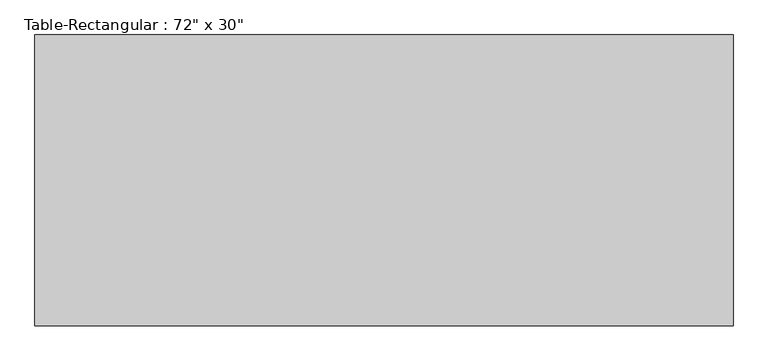
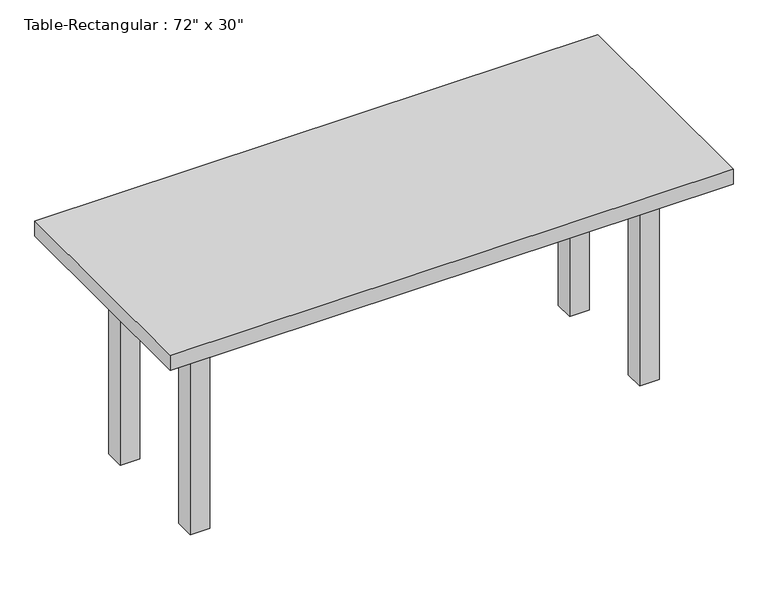
"""IFC4 building model written with IfcOpenShell, lengths in millimetres: furniture geometry."""

import ifcopenshell
import ifcopenshell.guid

model = None  # the IFC model being written
_history = None  # IfcOwnerHistory: only IFC2X3 demands one
_inside = {}  # id of a spatial element -> (the spatial element, [elements in it])
_under = {}  # id of a project, library or spatial element -> (it, [spatial elements below it])
_declared = {}  # id of a project -> (the project, [libraries it declares])
_typed = {}  # id of a type object -> (the type object, [elements of that type])
_made_of = {}  # id of a material, layer set ... -> (it, [elements and type objects made of it])


def new_model(schema):
    """Start an empty IFC model of exactly this schema.

    Asked for "IFC4X3", IfcOpenShell would pick the latest addendum, in which some entities
    have other attributes; the version numbers below select the first issue.
    IFC2X3 requires an IfcOwnerHistory on every rooted entity: one is made here for all.
    """
    global model, _history
    if schema == "IFC4X3":
        model = ifcopenshell.file(schema_version=(4, 3, 0, 0))
    else:
        model = ifcopenshell.file(schema=schema)
    _inside.clear()
    _under.clear()
    _declared.clear()
    _typed.clear()
    _made_of.clear()
    _history = None
    if model.schema == "IFC2X3":
        org = make("IfcOrganization", Name="unknown")
        user = make(
            "IfcPersonAndOrganization",
            ThePerson=make("IfcPerson", FamilyName="unknown"),
            TheOrganization=org,
        )
        app = make(
            "IfcApplication",
            ApplicationDeveloper=org,
            Version="unknown",
            ApplicationFullName="unknown",
            ApplicationIdentifier="unknown",
        )
        _history = make(
            "IfcOwnerHistory",
            OwningUser=user,
            OwningApplication=app,
            ChangeAction="ADDED",
            CreationDate=0,
        )
    return model


def make(cls, **values):
    """One entity of the class cls with the attributes given. An attribute that is None is left unset."""
    return model.create_entity(
        cls, **{name: value for name, value in values.items() if value is not None}
    )


def rooted(cls, **values):
    """An entity with a GlobalId (a new one), such as an element, a storey or a relation."""
    return make(cls, GlobalId=ifcopenshell.guid.new(), OwnerHistory=_history, **values)


def si_unit(unit_type, name, prefix=None):
    """IfcSIUnit, for example si_unit("LENGTHUNIT", "METRE", prefix="MILLI")."""
    return make("IfcSIUnit", UnitType=unit_type, Prefix=prefix, Name=name)


def assignment(units):
    """IfcUnitAssignment: the units of a project."""
    return None if units is None else make("IfcUnitAssignment", Units=units)


def point(xyz):
    """IfcCartesianPoint."""
    return None if xyz is None else make("IfcCartesianPoint", Coordinates=xyz)


def direction(xyz):
    """IfcDirection."""
    return None if xyz is None else make("IfcDirection", DirectionRatios=xyz)


def frame(location, z_axis=None, x_axis=None):
    """IfcAxis2Placement3D, a coordinate frame: its origin and axes. An axis left out is left unset."""
    return make(
        "IfcAxis2Placement3D",
        Location=point(location),
        Axis=direction(z_axis),
        RefDirection=direction(x_axis),
    )


def origin():
    """The frame at (0, 0, 0) with its axes left unset."""
    return frame((0.0, 0.0, 0.0))


def origin_with_axes():
    """The frame at (0, 0, 0) with the z axis (0, 0, 1) and the x axis (1, 0, 0) written out."""
    return frame((0.0, 0.0, 0.0), z_axis=(0.0, 0.0, 1.0), x_axis=(1.0, 0.0, 0.0))


def place(relative_to, where):
    """IfcLocalPlacement: puts the frame where relative to a parent placement (None: the world)."""
    return make(
        "IfcLocalPlacement", PlacementRelTo=relative_to, RelativePlacement=where
    )


def context(
    kind, dimensions, precision=None, world=None, true_north=None, identifier=None
):
    """IfcGeometricRepresentationContext, for example the 3D "Model" context."""
    return make(
        "IfcGeometricRepresentationContext",
        ContextIdentifier=identifier,
        ContextType=kind,
        CoordinateSpaceDimension=dimensions,
        Precision=precision,
        WorldCoordinateSystem=world,
        TrueNorth=true_north,
    )


def project(units=None, contexts=None):
    """IfcProject with its units and contexts."""
    return rooted(
        "IfcProject",
        Name="project",
        RepresentationContexts=contexts,
        UnitsInContext=assignment(units),
    )


def spatial(cls, under=None, at=None, **own):
    """A site, building, storey or space (cls), placed at a placement, below another one or the project."""
    s = rooted(cls, ObjectPlacement=at, **own)
    if under is not None:
        _under.setdefault(under.id(), (under, []))[1].append(s)
    return s


def polyline(points):
    """IfcPolyline through the points."""
    return make("IfcPolyline", Points=[point(p) for p in points])


def outline(outer, holes=None, kind="AREA"):
    """IfcArbitraryClosedProfileDef: a profile drawn as a closed curve; with holes, ...WithVoids."""
    if holes is None:
        return make("IfcArbitraryClosedProfileDef", ProfileType=kind, OuterCurve=outer)
    return make(
        "IfcArbitraryProfileDefWithVoids",
        ProfileType=kind,
        OuterCurve=outer,
        InnerCurves=holes,
    )


def extrude(swept, where, along, depth):
    """IfcExtrudedAreaSolid: the profile swept, set in the frame where, extruded along a direction by depth."""
    return make(
        "IfcExtrudedAreaSolid",
        SweptArea=swept,
        Position=where,
        ExtrudedDirection=direction(along),
        Depth=depth,
    )


def shape(context_of_items, identifier, shape_type, items):
    """IfcShapeRepresentation: the items that make up one representation, for example the "Body"."""
    return make(
        "IfcShapeRepresentation",
        ContextOfItems=context_of_items,
        RepresentationIdentifier=identifier,
        RepresentationType=shape_type,
        Items=items,
    )


def source(mapping_origin, context_of_items, identifier, shape_type, items):
    """IfcRepresentationMap: a shape defined once, which mapped items show again and again."""
    return make(
        "IfcRepresentationMap",
        MappingOrigin=mapping_origin,
        MappedRepresentation=shape(context_of_items, identifier, shape_type, items),
    )


def transform(
    local_origin,
    x_axis=None,
    y_axis=None,
    z_axis=None,
    scale=None,
    scale2=None,
    scale3=None,
    uniform=True,
):
    """IfcCartesianTransformationOperator3D, or its non-uniform kind. x_axis, y_axis, z_axis: its Axis1, 2, 3."""
    if uniform:
        return make(
            "IfcCartesianTransformationOperator3D",
            Axis1=direction(x_axis),
            Axis2=direction(y_axis),
            LocalOrigin=point(local_origin),
            Scale=scale,
            Axis3=direction(z_axis),
        )
    return make(
        "IfcCartesianTransformationOperator3DnonUniform",
        Axis1=direction(x_axis),
        Axis2=direction(y_axis),
        LocalOrigin=point(local_origin),
        Scale=scale,
        Axis3=direction(z_axis),
        Scale2=scale2,
        Scale3=scale3,
    )


def mapped(mapping_source, mapping_target):
    """IfcMappedItem: shows the shape of a source again, moved by a transform."""
    return make(
        "IfcMappedItem", MappingSource=mapping_source, MappingTarget=mapping_target
    )


def made_of(thing, what):
    """Note that an element or type object is made of a material, layer set ...; save() writes the relation."""
    if what is not None:
        _made_of.setdefault(what.id(), (what, []))[1].append(thing)
    return thing


def element(
    cls,
    number,
    at=None,
    inside=None,
    cuts=None,
    type_object=None,
    material=None,
    context=None,
    identifier="Body",
    shape_type=None,
    held_by="IfcProductDefinitionShape",
    body=None,
    shapes=None,
    **own,
):
    """One element of the class cls, such as IfcWall. Its Tag is "e" and its number.

    at: its placement. inside: the storey or other place that contains it. cuts: it is an
    opening in that element (IfcRelVoidsElement). A single representation is given by context,
    identifier, shape_type and body (its items); several are given by shapes. held_by: the class
    of the entity that holds the representations. save() writes the other relations.
    """
    e = rooted(cls, Tag="e%d" % number, ObjectPlacement=at, **own)
    if body is not None:
        shapes = [shape(context, identifier, shape_type, body)]
    if shapes is not None:
        e.Representation = make(held_by, Representations=shapes)
    if inside is not None:
        _inside.setdefault(inside.id(), (inside, []))[1].append(e)
    if cuts is not None:
        rooted(
            "IfcRelVoidsElement", RelatingBuildingElement=cuts, RelatedOpeningElement=e
        )
    if type_object is not None:
        _typed.setdefault(type_object.id(), (type_object, []))[1].append(e)
    return made_of(e, material)


def aggregate(whole, parts):
    """IfcRelAggregates: a whole, such as a stair, and the parts it consists of."""
    return rooted("IfcRelAggregates", RelatingObject=whole, RelatedObjects=parts)


def save(model, path):
    """Write the relations noted so far, then the file.

    IfcRelAggregates (storeys below a building ...), IfcRelContainedInSpatialStructure (elements
    in a storey), IfcRelDefinesByType, IfcRelAssociatesMaterial and IfcRelDeclares: one each for
    every whole, place, type object, material and project.
    """
    for whole, parts in _under.values():
        aggregate(whole, parts)
    for where, things in _inside.values():
        rooted(
            "IfcRelContainedInSpatialStructure",
            RelatedElements=things,
            RelatingStructure=where,
        )
    for kind, things in _typed.values():
        rooted("IfcRelDefinesByType", RelatedObjects=things, RelatingType=kind)
    for what, things in _made_of.values():
        rooted("IfcRelAssociatesMaterial", RelatedObjects=things, RelatingMaterial=what)
    for by, libraries in _declared.values():
        rooted("IfcRelDeclares", RelatingContext=by, RelatedDefinitions=libraries)
    model.write(path)


def furniture_a5b052b6(model_context):
    return source(origin(), model_context, "Body", "SweptSolid", [
        extrude(outline(polyline([(698.5, 190.5), (698.5, 165.1), (-698.5, 165.1), (-698.5, 190.5), (698.5, 190.5)])), frame((0.0, 0.0, 609.6), z_axis=(0.0, 0.0, 1.0), x_axis=(1.0, 0.0, 0.0)), (0.0, 0.0, 1.0), 101.6),
        extrude(outline(polyline([(698.5, -190.5), (-698.5, -190.5), (-698.5, -165.1), (698.5, -165.1), (698.5, -190.5)])), frame((0.0, 0.0, 609.6), z_axis=(0.0, 0.0, 1.0), x_axis=(1.0, 0.0, 0.0)), (0.0, 0.0, 1.0), 101.6),
        extrude(outline(polyline([(-711.2, -165.1), (-736.6, -165.1), (-736.6, 165.1), (-711.2, 165.1), (-711.2, -165.1)])), frame((0.0, 0.0, 609.6), z_axis=(0.0, 0.0, 1.0), x_axis=(1.0, 0.0, 0.0)), (0.0, 0.0, 1.0), 101.6),
        extrude(outline(polyline([(711.2, -165.1), (711.2, 165.1), (736.6, 165.1), (736.6, -165.1), (711.2, -165.1)])), frame((0.0, 0.0, 609.6), z_axis=(0.0, 0.0, 1.0), x_axis=(1.0, 0.0, 0.0)), (0.0, 0.0, 1.0), 101.6),
        extrude(outline(polyline([(914.4, 381.0), (914.4, -381.0), (-914.4, -381.0), (-914.4, 381.0), (914.4, 381.0)])), frame((0.0, 0.0, 711.2), z_axis=(0.0, 0.0, 1.0), x_axis=(1.0, 0.0, 0.0)), (0.0, 0.0, 1.0), 50.8),
        extrude(outline(polyline([(-698.5, 228.6), (-698.5, 165.1), (-762.0, 165.1), (-762.0, 228.6), (-698.5, 228.6)])), origin_with_axes(), (0.0, 0.0, 1.0), 711.2),
        extrude(outline(polyline([(698.5, 228.6), (762.0, 228.6), (762.0, 165.1), (698.5, 165.1), (698.5, 228.6)])), origin_with_axes(), (0.0, 0.0, 1.0), 711.2),
        extrude(outline(polyline([(-698.5, -228.6), (-762.0, -228.6), (-762.0, -165.1), (-698.5, -165.1), (-698.5, -228.6)])), origin_with_axes(), (0.0, 0.0, 1.0), 711.2),
        extrude(outline(polyline([(698.5, -228.6), (698.5, -165.1), (762.0, -165.1), (762.0, -228.6), (698.5, -228.6)])), origin_with_axes(), (0.0, 0.0, 1.0), 711.2),
    ])


if __name__ == "__main__":
    model = new_model("IFC4")
    model_context = context("Model", 3, world=origin())
    ifc_project = project(units=[si_unit("LENGTHUNIT", "METRE", prefix="MILLI")], contexts=[model_context])
    site = spatial("IfcSite", under=ifc_project)
    building = spatial("IfcBuilding", under=site)
    placement = place(None, origin())
    furniture_shape = furniture_a5b052b6(model_context)
    element("IfcFurniture", 1, ObjectType="Table-Rectangular : 72\" x 30\"", at=placement, inside=building, context=model_context, shape_type="MappedRepresentation", body=[
        mapped(furniture_shape, transform((0.0, 0.0, 0.0), x_axis=(1.0, 0.0, 0.0), y_axis=(0.0, 1.0, 0.0), z_axis=(0.0, 0.0, 1.0))),
    ])
    save(model, "model.ifc")

# Revit data of these elements
# Type "Table-Rectangular : 72\" x 30\""
#   Assembly Code = "E2020200"
#   Height = 2' - 6"
#   Length = 6' - 0"
#   Width = 2' - 6"
#   Base Material = Birch
#   Top Material = Birch
#   Default Elevation = 0
# Element 1 (IfcFurniture, "Table-Rectangular : 72\" x 30\"")
#   Materials on its faces: "Birch"
# Materials
#   "Birch": class "Wood", colour RGB 224 178 126, transparency 0, Description = "Betula Alleghaniensis", Cost = 0
